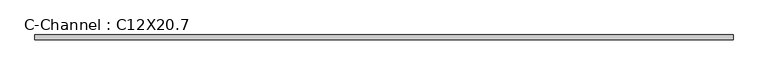
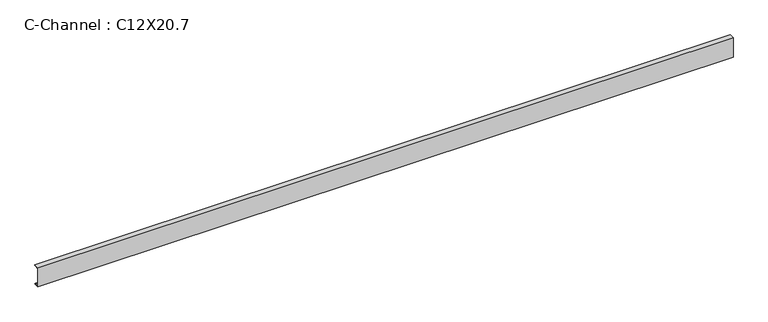
"""IFC4 building model written with IfcOpenShell, lengths in millimetres: beam geometry, C-Channel : C12X20.7."""

from ifc_helpers import new_model, si_unit, point, frame, frame_2d, origin, place, context, project, spatial, polyline, circle_curve, trimmed, segment, composite_curve, outline, extrude, source, transform, mapped, element, save


def c_channel_c12x20_7_e832e308(model_context):
    return source(origin(), model_context, "Body", "SweptSolid", [
        extrude(outline(composite_curve([segment(polyline([(-17.7292, 152.4), (56.9468, 152.4)]), True, "CONTINUOUS"), segment(trimmed(circle_curve(frame_2d((44.2214, 152.4)), 12.7254), [point((56.9468, 152.4))], [point((44.2214, 139.6746))], False, "CARTESIAN"), True, "CONTINUOUS"), segment(polyline([(44.2214, 139.6746), (-10.5664, 130.997065), (-10.5664, -130.997065), (44.2214, -139.6746)]), True, "CONTINUOUS"), segment(trimmed(circle_curve(frame_2d((44.2214, -152.4)), 12.7254), [point((44.2214, -139.6746))], [point((56.9468, -152.4))], False, "CARTESIAN"), True, "CONTINUOUS"), segment(polyline([(56.9468, -152.4), (-17.7292, -152.4), (-17.7292, 152.4)]), True, "CONTINUOUS")], self_intersect=False)), frame((-5203.4337987, 0.0, 0.0), z_axis=(1.0, 0.0, 0.0), x_axis=(0.0, 1.0, 0.0)), (0.0, 0.0, 1.0), 10410.7769404),
    ])


if __name__ == "__main__":
    model = new_model("IFC4")
    model_context = context("Model", 3, world=origin())
    ifc_project = project(units=[si_unit("LENGTHUNIT", "METRE", prefix="MILLI")], contexts=[model_context])
    site = spatial("IfcSite", under=ifc_project)
    building = spatial("IfcBuilding", under=site)
    placement = place(None, origin())
    c_channel_c12x20_7_shape = c_channel_c12x20_7_e832e308(model_context)
    element("IfcBeam", 1, ObjectType="C-Channel : C12X20.7", at=placement, inside=building, context=model_context, shape_type="MappedRepresentation", body=[
        mapped(c_channel_c12x20_7_shape, transform((0.0, 0.0, 0.0), x_axis=(1.0, 0.0, 0.0), y_axis=(0.0, 1.0, 0.0), z_axis=(0.0, 0.0, 1.0))),
    ])
    save(model, "model.ifc")

# Revit data of these elements
# Type "C-Channel : C12X20.7"
#   Assembly Code = "B10"
#   W = 20.7
#   Start Extension Calculation [instance default] = 10' - 0"
#   Start Extension [instance default] = -0' - 0 1/2"
#   End Extension Calculation [instance default] = 10' - 0"
#   End Extension [instance default] = -0' - 0 1/2"
#   Length [instance default] = 5' - 0"
#   bf = 0' - 2.94"
#   d = 1' - 0"
#   tf = 0' - 0.501"
#   tw = 0' - 0.282"
#   x = 0' - 0.698"
#   A = 0.0422222 SF
#   Structural Material [instance default] = Metal - Steel - ASTM A36
# Element 1 (IfcBeam, "C-Channel : C12X20.7")
#   Materials on its faces: "Metal - Steel - ASTM A36"
# Materials
#   "Metal - Steel - ASTM A36": class "Metal", colour RGB 199 199 199, transparency 0
